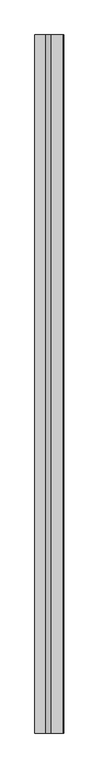
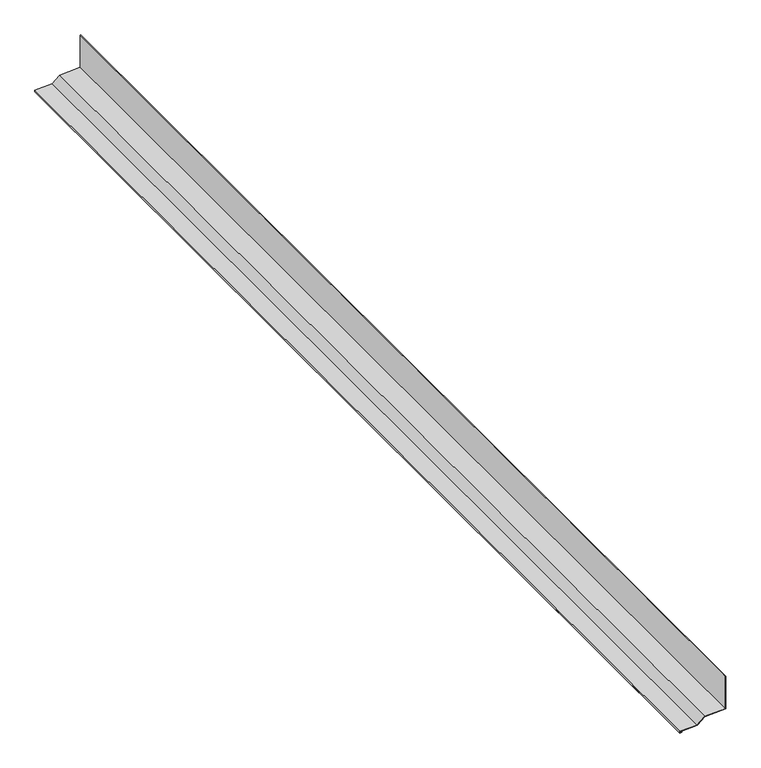
"""IFC4 building model written with IfcOpenShell, lengths in millimetres: proxy geometry, Generic Models 7:Generic Models 1:337419:Generic Models 1:337419 : Generic Models 7:Generic Models 1:337419:28 : Generic Models 7:Generic Models 1:337419:Generic Models 1:337419 : Generic Models 7:Generic Models 1:337419:301336."""

from ifc_helpers import new_model, si_unit, frame, origin, place, context, project, spatial, polyline, outline, extrude, source, transform, mapped, element, save


def generic_models_1712cdd1(model_context):
    return source(origin(), model_context, "Body", "SweptSolid", [
        extrude(outline(polyline([(4816.1034977, 579102.924224), (4812.9312502, 579026.7902838), (4788.4410423, 578997.6039905), (4785.7975027, 578934.1590404), (4779.4530077, 578934.4233943), (4779.7561986, 578941.6999752), (4781.345076, 578941.6999752), (4781.10522, 578935.9434296), (4784.2774675, 578935.8112526), (4786.877426, 578998.2102567), (4811.3676339, 579027.39655), (4814.5807661, 579104.511724), (4943.1034977, 579104.511724), (4943.1034977, 579102.924224), (4816.1034977, 579102.924224)])), frame((0.0, -578797.4913841, 0.0), z_axis=(0.0, 1.0, 0.0), x_axis=(0.0, 0.0, 1.0)), (0.0, 0.0, 1.0), 4145.5624605),
    ])


if __name__ == "__main__":
    model = new_model("IFC4")
    model_context = context("Model", 3, world=origin())
    ifc_project = project(units=[si_unit("LENGTHUNIT", "METRE", prefix="MILLI")], contexts=[model_context])
    site = spatial("IfcSite", under=ifc_project)
    building = spatial("IfcBuilding", under=site)
    placement = place(None, origin())
    generic_models_shape = generic_models_1712cdd1(model_context)
    element("IfcBuildingElementProxy", 1, Name="Generic Models 7:Generic Models 1:337419:Generic Models 1:337419 : Generic Models 7:Generic Models 1:337419:28 : Generic Models 7:Generic Models 1:337419:Generic Models 1:337419 : Generic Models 7:Generic Models 1:337419:301336", ObjectType="Generic Models 7:Generic Models 1:337419:Generic Models 1:337419 : Generic Models 7:Generic Models 1:337419:28 : Generic Models 7:Generic Models 1:337419:Generic Models 1:337419 : Generic Models 7:Generic Models 1:337419:301336", at=placement, inside=building, context=model_context, shape_type="MappedRepresentation", body=[
        mapped(generic_models_shape, transform((0.0, 0.0, 0.0), x_axis=(1.0, 0.0, 0.0), y_axis=(0.0, 1.0, 0.0), z_axis=(0.0, 0.0, 1.0))),
    ])
    save(model, "model.ifc")

# Revit data of these elements
# Type "Generic Models 7:Generic Models 1:337419:Generic Models 1:337419 : Generic Models 7:Generic Models 1:337419:28 : Generic Models 7:Generic Models 1:337419:Generic Models 1:337419 : Generic Models 7:Generic Models 1:337419:301336"
#   NameOverride = "Generic Models 7:Generic Models 1:337419:Generic Models 1:337419 : Generic Models 7:Generic Models 1:337419:301336"
#   ObjectTypeOverride = "Generic Models 1:337419 : Generic Models 7:Generic Models 1:337419"
#   Reference = "Generic Models 1"
#   Tag = "301336"
# Element 1 (IfcBuildingElementProxy, "Generic Models 7:Generic Models 1:337419:Generic Models 1:337419 : Generic Models 7:Generic Models 1:337419:28 : Generic Models 7:Generic Models 1:337419:Generic Models 1:337419 : Generic Models 7:Generic Models 1:337419:301336")
#   Materials on its faces: "PARAPET HIGH EAVE TRIM"
# Materials
#   "PARAPET HIGH EAVE TRIM": class "Unassigned", colour RGB 182 182 182, transparency 0, Cost = 0
